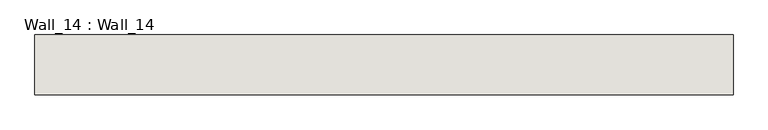
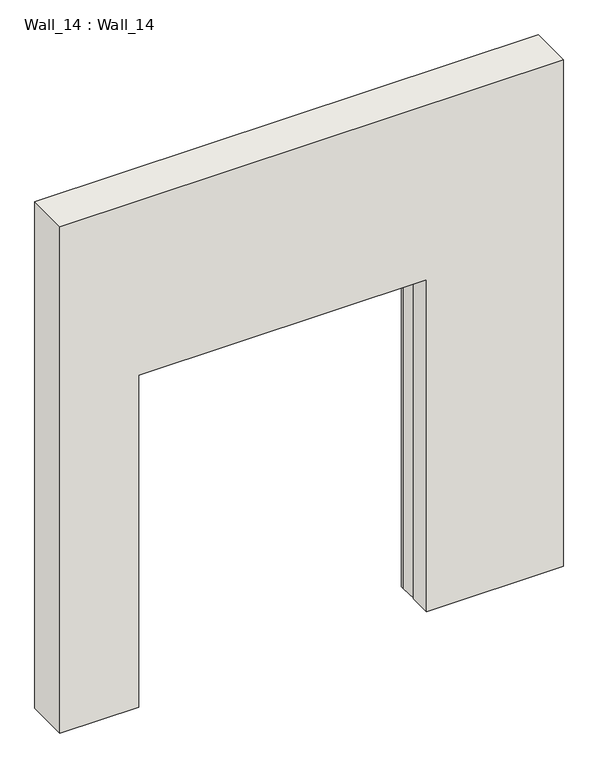
"""IFC4 building model written with IfcOpenShell, lengths in millimetres: wall geometry, Wall_14 : Wall_14."""

from ifc_helpers import new_model, si_unit, origin, place, context, project, spatial, faceted_brep, source, transform, mapped, element, save


def wall_14_wall_14_043e5d1d(model_context):
    return source(origin(), model_context, "Body", "Brep", [
        faceted_brep([(4660.0, 0.0, 4700.0), (4660.0, 380.0, 4700.0), (240.0, 380.0, 4700.0), (240.0, 0.0, 4700.0), (240.0, 0.0, 0.0), (240.0, 380.0, 0.0), (926.5217391, 380.0, 0.0), (930.0, 270.0, 0.0), (930.0, 0.0, 0.0), (4660.0, 380.0, 0.0), (4660.0, 0.0, 0.0), (3460.0, 0.0, 0.0), (3460.0, 199.9250293, 0.0), (3464.7407136, 200.0749333, 0.0), (3460.0, 350.0, 0.0), (3460.0, 380.0, 0.0), (3460.0, 380.0, 3080.0), (3459.0513834, 380.0, 3080.0), (3459.0513834, 380.0, 4050.0), (926.5217391, 380.0, 4050.0), (930.0, 0.0, 3080.0), (3460.0, 0.0, 3080.0), (3464.7407136, 200.0749333, 4050.0), (934.7407136, 120.0749333, 4050.0), (3460.0, 350.0, 3080.0), (934.7407136, 120.0749333, 3080.0), (930.0, 270.0, 3080.0), (3460.0, 199.9250293, 3080.0)], [[[0, 1, 2, 3]], [[4, 5, 6, 7, 8]], [[9, 10, 11, 12, 13, 14, 15]], [[1, 0, 10, 9]], [[2, 1, 9, 15, 16, 17, 18, 19, 6, 5]], [[3, 2, 5, 4]], [[0, 3, 4, 8, 20, 21, 11, 10]], [[22, 23, 19, 18]], [[13, 22, 18, 17, 24, 14]], [[19, 23, 25, 26, 7, 6]], [[23, 22, 13, 12, 27, 25]], [[20, 26, 25, 27, 21]], [[16, 24, 17]], [[21, 27, 12, 11]], [[24, 16, 15, 14]], [[26, 20, 8, 7]]]),
    ])


if __name__ == "__main__":
    model = new_model("IFC4")
    model_context = context("Model", 3, world=origin())
    ifc_project = project(units=[si_unit("LENGTHUNIT", "METRE", prefix="MILLI")], contexts=[model_context])
    site = spatial("IfcSite", under=ifc_project)
    building = spatial("IfcBuilding", under=site)
    placement = place(None, origin())
    wall_14_wall_14_shape = wall_14_wall_14_043e5d1d(model_context)
    element("IfcWall", 1, ObjectType="Wall_14 : Wall_14", at=placement, inside=building, context=model_context, shape_type="MappedRepresentation", body=[
        mapped(wall_14_wall_14_shape, transform((0.0, 0.0, 0.0), x_axis=(1.0, 0.0, 0.0), y_axis=(0.0, 1.0, 0.0), z_axis=(0.0, 0.0, 1.0))),
    ])
    save(model, "model.ifc")

# Revit data of these elements
# Type "Wall_14 : Wall_14"
#   NameOverride = "Wall_14"
# Element 1 (IfcWall, "Wall_14 : Wall_14")
#   Materials on its faces: "IfcSurfaceStyle #33"
# Materials
#   "IfcSurfaceStyle #33": class "Unassigned", colour RGB 214 214 214, transparency 0
